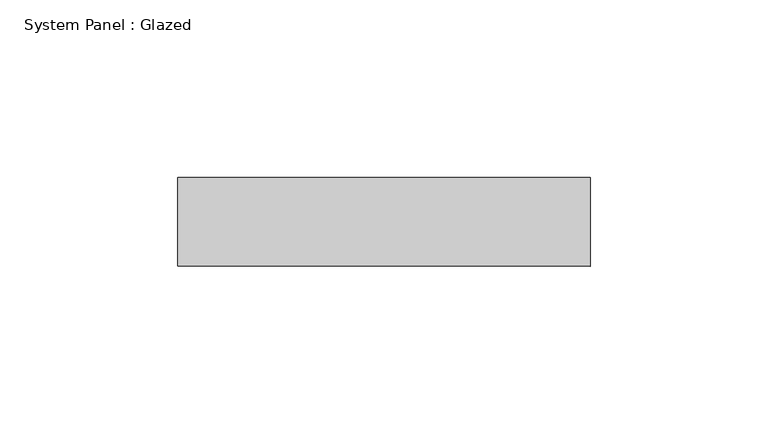
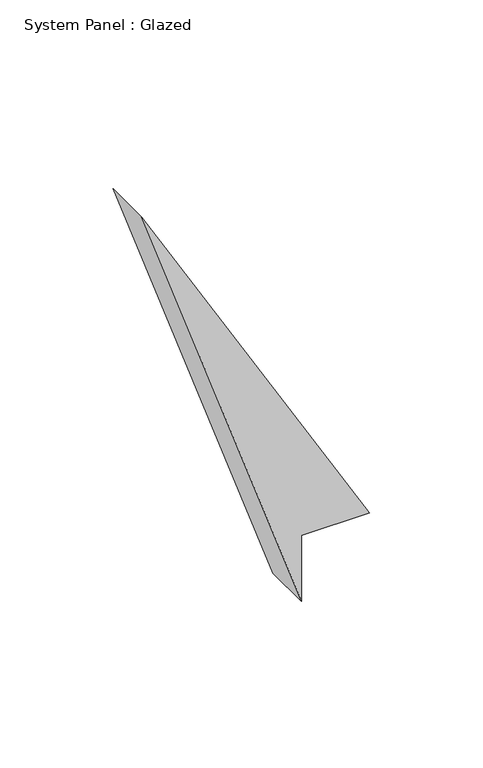
"""IFC4 building model written with IfcOpenShell, lengths in millimetres: plate geometry, System Panel : Glazed."""

import ifcopenshell
import ifcopenshell.guid

model = None  # the IFC model being written
_history = None  # IfcOwnerHistory: only IFC2X3 demands one
_inside = {}  # id of a spatial element -> (the spatial element, [elements in it])
_under = {}  # id of a project, library or spatial element -> (it, [spatial elements below it])
_declared = {}  # id of a project -> (the project, [libraries it declares])
_typed = {}  # id of a type object -> (the type object, [elements of that type])
_made_of = {}  # id of a material, layer set ... -> (it, [elements and type objects made of it])


def new_model(schema):
    """Start an empty IFC model of exactly this schema.

    Asked for "IFC4X3", IfcOpenShell would pick the latest addendum, in which some entities
    have other attributes; the version numbers below select the first issue.
    IFC2X3 requires an IfcOwnerHistory on every rooted entity: one is made here for all.
    """
    global model, _history
    if schema == "IFC4X3":
        model = ifcopenshell.file(schema_version=(4, 3, 0, 0))
    else:
        model = ifcopenshell.file(schema=schema)
    _inside.clear()
    _under.clear()
    _declared.clear()
    _typed.clear()
    _made_of.clear()
    _history = None
    if model.schema == "IFC2X3":
        org = make("IfcOrganization", Name="unknown")
        user = make(
            "IfcPersonAndOrganization",
            ThePerson=make("IfcPerson", FamilyName="unknown"),
            TheOrganization=org,
        )
        app = make(
            "IfcApplication",
            ApplicationDeveloper=org,
            Version="unknown",
            ApplicationFullName="unknown",
            ApplicationIdentifier="unknown",
        )
        _history = make(
            "IfcOwnerHistory",
            OwningUser=user,
            OwningApplication=app,
            ChangeAction="ADDED",
            CreationDate=0,
        )
    return model


def make(cls, **values):
    """One entity of the class cls with the attributes given. An attribute that is None is left unset."""
    return model.create_entity(
        cls, **{name: value for name, value in values.items() if value is not None}
    )


def rooted(cls, **values):
    """An entity with a GlobalId (a new one), such as an element, a storey or a relation."""
    return make(cls, GlobalId=ifcopenshell.guid.new(), OwnerHistory=_history, **values)


def si_unit(unit_type, name, prefix=None):
    """IfcSIUnit, for example si_unit("LENGTHUNIT", "METRE", prefix="MILLI")."""
    return make("IfcSIUnit", UnitType=unit_type, Prefix=prefix, Name=name)


def assignment(units):
    """IfcUnitAssignment: the units of a project."""
    return None if units is None else make("IfcUnitAssignment", Units=units)


def point(xyz):
    """IfcCartesianPoint."""
    return None if xyz is None else make("IfcCartesianPoint", Coordinates=xyz)


def direction(xyz):
    """IfcDirection."""
    return None if xyz is None else make("IfcDirection", DirectionRatios=xyz)


def frame(location, z_axis=None, x_axis=None):
    """IfcAxis2Placement3D, a coordinate frame: its origin and axes. An axis left out is left unset."""
    return make(
        "IfcAxis2Placement3D",
        Location=point(location),
        Axis=direction(z_axis),
        RefDirection=direction(x_axis),
    )


def origin():
    """The frame at (0, 0, 0) with its axes left unset."""
    return frame((0.0, 0.0, 0.0))


def place(relative_to, where):
    """IfcLocalPlacement: puts the frame where relative to a parent placement (None: the world)."""
    return make(
        "IfcLocalPlacement", PlacementRelTo=relative_to, RelativePlacement=where
    )


def context(
    kind, dimensions, precision=None, world=None, true_north=None, identifier=None
):
    """IfcGeometricRepresentationContext, for example the 3D "Model" context."""
    return make(
        "IfcGeometricRepresentationContext",
        ContextIdentifier=identifier,
        ContextType=kind,
        CoordinateSpaceDimension=dimensions,
        Precision=precision,
        WorldCoordinateSystem=world,
        TrueNorth=true_north,
    )


def project(units=None, contexts=None):
    """IfcProject with its units and contexts."""
    return rooted(
        "IfcProject",
        Name="project",
        RepresentationContexts=contexts,
        UnitsInContext=assignment(units),
    )


def spatial(cls, under=None, at=None, **own):
    """A site, building, storey or space (cls), placed at a placement, below another one or the project."""
    s = rooted(cls, ObjectPlacement=at, **own)
    if under is not None:
        _under.setdefault(under.id(), (under, []))[1].append(s)
    return s


def polyline(points):
    """IfcPolyline through the points."""
    return make("IfcPolyline", Points=[point(p) for p in points])


def outline(outer, holes=None, kind="AREA"):
    """IfcArbitraryClosedProfileDef: a profile drawn as a closed curve; with holes, ...WithVoids."""
    if holes is None:
        return make("IfcArbitraryClosedProfileDef", ProfileType=kind, OuterCurve=outer)
    return make(
        "IfcArbitraryProfileDefWithVoids",
        ProfileType=kind,
        OuterCurve=outer,
        InnerCurves=holes,
    )


def extrude(swept, where, along, depth):
    """IfcExtrudedAreaSolid: the profile swept, set in the frame where, extruded along a direction by depth."""
    return make(
        "IfcExtrudedAreaSolid",
        SweptArea=swept,
        Position=where,
        ExtrudedDirection=direction(along),
        Depth=depth,
    )


def shape(context_of_items, identifier, shape_type, items):
    """IfcShapeRepresentation: the items that make up one representation, for example the "Body"."""
    return make(
        "IfcShapeRepresentation",
        ContextOfItems=context_of_items,
        RepresentationIdentifier=identifier,
        RepresentationType=shape_type,
        Items=items,
    )


def source(mapping_origin, context_of_items, identifier, shape_type, items):
    """IfcRepresentationMap: a shape defined once, which mapped items show again and again."""
    return make(
        "IfcRepresentationMap",
        MappingOrigin=mapping_origin,
        MappedRepresentation=shape(context_of_items, identifier, shape_type, items),
    )


def transform(
    local_origin,
    x_axis=None,
    y_axis=None,
    z_axis=None,
    scale=None,
    scale2=None,
    scale3=None,
    uniform=True,
):
    """IfcCartesianTransformationOperator3D, or its non-uniform kind. x_axis, y_axis, z_axis: its Axis1, 2, 3."""
    if uniform:
        return make(
            "IfcCartesianTransformationOperator3D",
            Axis1=direction(x_axis),
            Axis2=direction(y_axis),
            LocalOrigin=point(local_origin),
            Scale=scale,
            Axis3=direction(z_axis),
        )
    return make(
        "IfcCartesianTransformationOperator3DnonUniform",
        Axis1=direction(x_axis),
        Axis2=direction(y_axis),
        LocalOrigin=point(local_origin),
        Scale=scale,
        Axis3=direction(z_axis),
        Scale2=scale2,
        Scale3=scale3,
    )


def mapped(mapping_source, mapping_target):
    """IfcMappedItem: shows the shape of a source again, moved by a transform."""
    return make(
        "IfcMappedItem", MappingSource=mapping_source, MappingTarget=mapping_target
    )


def made_of(thing, what):
    """Note that an element or type object is made of a material, layer set ...; save() writes the relation."""
    if what is not None:
        _made_of.setdefault(what.id(), (what, []))[1].append(thing)
    return thing


def element(
    cls,
    number,
    at=None,
    inside=None,
    cuts=None,
    type_object=None,
    material=None,
    context=None,
    identifier="Body",
    shape_type=None,
    held_by="IfcProductDefinitionShape",
    body=None,
    shapes=None,
    **own,
):
    """One element of the class cls, such as IfcWall. Its Tag is "e" and its number.

    at: its placement. inside: the storey or other place that contains it. cuts: it is an
    opening in that element (IfcRelVoidsElement). A single representation is given by context,
    identifier, shape_type and body (its items); several are given by shapes. held_by: the class
    of the entity that holds the representations. save() writes the other relations.
    """
    e = rooted(cls, Tag="e%d" % number, ObjectPlacement=at, **own)
    if body is not None:
        shapes = [shape(context, identifier, shape_type, body)]
    if shapes is not None:
        e.Representation = make(held_by, Representations=shapes)
    if inside is not None:
        _inside.setdefault(inside.id(), (inside, []))[1].append(e)
    if cuts is not None:
        rooted(
            "IfcRelVoidsElement", RelatingBuildingElement=cuts, RelatedOpeningElement=e
        )
    if type_object is not None:
        _typed.setdefault(type_object.id(), (type_object, []))[1].append(e)
    return made_of(e, material)


def aggregate(whole, parts):
    """IfcRelAggregates: a whole, such as a stair, and the parts it consists of."""
    return rooted("IfcRelAggregates", RelatingObject=whole, RelatedObjects=parts)


def save(model, path):
    """Write the relations noted so far, then the file.

    IfcRelAggregates (storeys below a building ...), IfcRelContainedInSpatialStructure (elements
    in a storey), IfcRelDefinesByType, IfcRelAssociatesMaterial and IfcRelDeclares: one each for
    every whole, place, type object, material and project.
    """
    for whole, parts in _under.values():
        aggregate(whole, parts)
    for where, things in _inside.values():
        rooted(
            "IfcRelContainedInSpatialStructure",
            RelatedElements=things,
            RelatingStructure=where,
        )
    for kind, things in _typed.values():
        rooted("IfcRelDefinesByType", RelatedObjects=things, RelatingType=kind)
    for what, things in _made_of.values():
        rooted("IfcRelAssociatesMaterial", RelatedObjects=things, RelatingMaterial=what)
    for by, libraries in _declared.values():
        rooted("IfcRelDeclares", RelatingContext=by, RelatedDefinitions=libraries)
    model.write(path)


def system_panel_glazed_54b3e94c(model_context):
    return source(origin(), model_context, "Body", "SweptSolid", [
        extrude(outline(polyline([(0.0, 23.3505759), (35.3553391, 23.3505759), (35.3553391, 58.0717743), (235.5388878, -58.0717743), (0.0, 23.3505759)])), frame((0.0, -49.5, 0.0), z_axis=(0.0, 1.0, 0.0), x_axis=(0.0, 0.0, 1.0)), (0.0, 0.0, 1.0), 25.0),
    ])


if __name__ == "__main__":
    model = new_model("IFC4")
    model_context = context("Model", 3, world=origin())
    ifc_project = project(units=[si_unit("LENGTHUNIT", "METRE", prefix="MILLI")], contexts=[model_context])
    site = spatial("IfcSite", under=ifc_project)
    building = spatial("IfcBuilding", under=site)
    placement = place(None, origin())
    system_panel_glazed_shape = system_panel_glazed_54b3e94c(model_context)
    element("IfcPlate", 1, ObjectType="System Panel : Glazed", at=placement, inside=building, context=model_context, shape_type="MappedRepresentation", body=[
        mapped(system_panel_glazed_shape, transform((0.0, 0.0, 0.0), x_axis=(1.0, 0.0, 0.0), y_axis=(0.0, 1.0, 0.0), z_axis=(0.0, 0.0, 1.0))),
    ])
    save(model, "model.ifc")

# Revit data of these elements
# Element 1 (IfcPlate, "System Panel : Glazed")
#   Materials on its faces: "Glass"
# Materials
#   "Glass": class "Glass", colour RGB 218 227 224, transparency 0.85, Description = "Soda Lime Glass", Cost = 0
